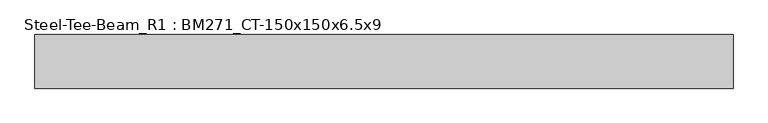
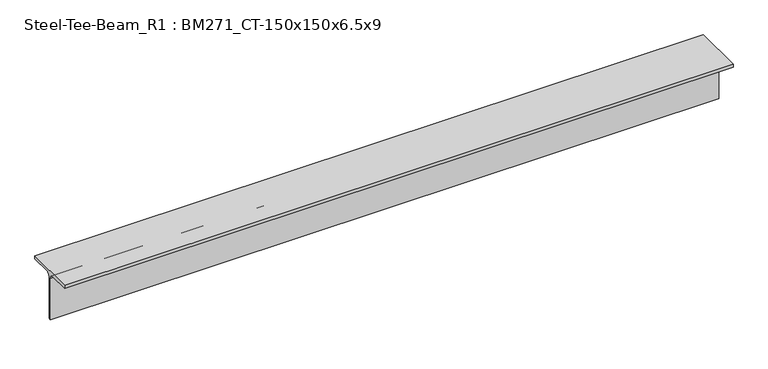
"""IFC4 building model written with IfcOpenShell, lengths in millimetres: member geometry, Steel-Tee-Beam_R1 : BM271_CT-150x150x6.5x9."""

from ifc_helpers import new_model, si_unit, point, frame, frame_2d, origin, place, context, project, spatial, polyline, circle_curve, trimmed, segment, composite_curve, outline, extrude, source, transform, mapped, element, save


def steel_tee_beam_r1_bm271_ct_150x150x6_5x9_a36b2b69(model_context):
    return source(origin(), model_context, "Body", "SweptSolid", [
        extrude(outline(composite_curve([segment(polyline([(-75.0, 75.0), (75.0, 75.0), (75.0, 66.0), (16.25, 66.0)]), True, "CONTINUOUS"), segment(trimmed(circle_curve(frame_2d((16.25, 53.0)), 13.0), [point((16.25, 66.0))], [point((3.25, 53.0))], True, "CARTESIAN"), True, "CONTINUOUS"), segment(polyline([(3.25, 53.0), (3.25, -75.0), (-3.25, -75.0), (-3.25, 53.0)]), True, "CONTINUOUS"), segment(trimmed(circle_curve(frame_2d((-16.25, 53.0)), 13.0), [point((-3.25, 53.0))], [point((-16.25, 66.0))], True, "CARTESIAN"), True, "CONTINUOUS"), segment(polyline([(-16.25, 66.0), (-75.0, 66.0), (-75.0, 75.0)]), True, "CONTINUOUS")], self_intersect=False)), frame((-983.9814396, 0.0, 0.0), z_axis=(1.0, 0.0, 0.0), x_axis=(0.0, 1.0, 0.0)), (0.0, 0.0, 1.0), 1951.2705213),
    ])


if __name__ == "__main__":
    model = new_model("IFC4")
    model_context = context("Model", 3, world=origin())
    ifc_project = project(units=[si_unit("LENGTHUNIT", "METRE", prefix="MILLI")], contexts=[model_context])
    site = spatial("IfcSite", under=ifc_project)
    building = spatial("IfcBuilding", under=site)
    placement = place(None, origin())
    steel_tee_beam_r1_bm271_ct_150x150x6_5x9_shape = steel_tee_beam_r1_bm271_ct_150x150x6_5x9_a36b2b69(model_context)
    element("IfcMember", 1, ObjectType="Steel-Tee-Beam_R1 : BM271_CT-150x150x6.5x9", at=placement, inside=building, context=model_context, shape_type="MappedRepresentation", body=[
        mapped(steel_tee_beam_r1_bm271_ct_150x150x6_5x9_shape, transform((0.0, 0.0, 0.0), x_axis=(1.0, 0.0, 0.0), y_axis=(0.0, 1.0, 0.0), z_axis=(0.0, 0.0, 1.0))),
    ])
    save(model, "model.ifc")

# Revit data of these elements
# Type "Steel-Tee-Beam_R1 : BM271_CT-150x150x6.5x9"
#   Keynote = "CT-150x150x6.5x9"
#   Surface Area = 0.588841 m²/m
#   Section Area = 23.3904 cm²
#   Mass per Unit Length = 18.3614 kg/m
#   Length [instance default] = 1.5240 m
#   bf = 0.1500 m
#   d = 0.1500 m
#   k = 0.0220 m
#   r = 0.0130 m
#   tf = 0.0090 m
#   tw = 0.0065 m
#   hec_material4 [instance default] = none
#   hec_material3 [instance default] = none
#   hec_material2 [instance default] = none
#   hec_material1 [instance default] = none
#   Structural Material [instance default] = Steel, 45-345
#   Assembly Code = ""
# Element 1 (IfcMember, "Steel-Tee-Beam_R1 : BM271_CT-150x150x6.5x9")
#   Structural Material = none
# Materials
#   "Steel, 45-345": class "Metal", colour RGB 189 187 185, transparency 0, Description = "Steel 345 MPa", Cost = 0
